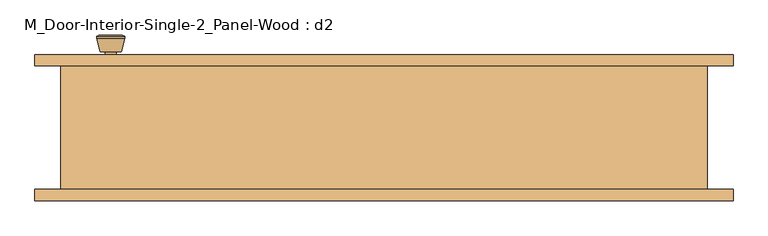
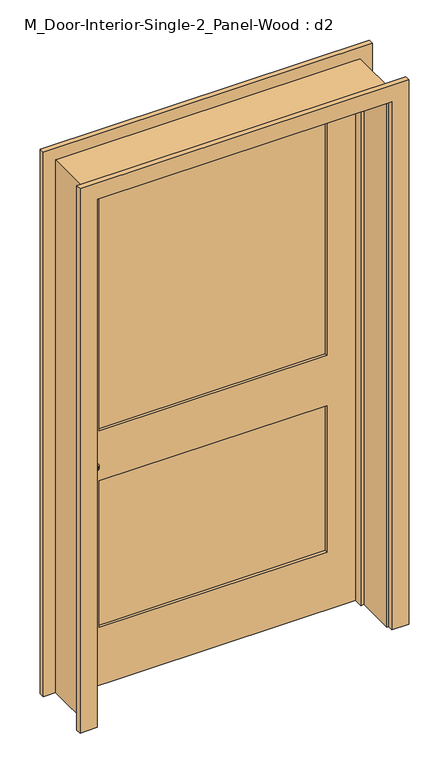
"""IFC4 building model written with IfcOpenShell, lengths in millimetres: door geometry, M_Door-Interior-Single-2_Panel-Wood : d2."""

from ifc_helpers import new_model, si_unit, point, frame, frame_2d, origin, place, context, project, spatial, polyline, circle_curve, trimmed, segment, composite_curve, outline, extrude, faceted_brep, source, transform, mapped, element, save
from ifc_brep_helpers import plane_surface, cylinder_surface, revolved_surface, advanced_brep


def m_door_interior_single_2_panel_wood_d2_7d5fc0ab(model_context):
    return source(origin(), model_context, "Body", "SolidModel", [
        advanced_brep(
        [(-486.5, 65.825, 914.4), (-476.5, 65.825, 914.4), (-496.5, 65.825, 914.4), (-466.0241324, 16.825, 914.4), (-486.5, 16.825, 914.4), (-506.9758676, 16.825, 914.4), (-461.5, 18.6528681, 914.4), (-511.5, 18.6528681, 914.4), (-461.5, 22.1165463, 914.4), (-511.5, 22.1165463, 914.4), (-467.863764, 46.825, 914.4), (-505.136236, 46.825, 914.4), (-476.5, 46.825, 914.4), (-496.5, 46.825, 914.4)],
        [
            (0, 1),
            (1, 2, circle_curve(frame((-486.5, 65.825, 914.4), z_axis=(0.0, 1.0, 0.0), x_axis=(-1.0, 0.0, 0.0)), 10.0)),
            (2, 0),
            (2, 1, circle_curve(frame((-486.5, 65.825, 914.4), z_axis=(0.0, 1.0, 0.0), x_axis=(-1.0, 0.0, 0.0)), 10.0)),
            (3, 4),
            (4, 5),
            (5, 3, circle_curve(frame((-486.5, 16.825, 914.4), z_axis=(0.0, -1.0, 0.0), x_axis=(-1.0, 0.0, 0.0)), 20.4758676)),
            (3, 5, circle_curve(frame((-486.5, 16.825, 914.4), z_axis=(0.0, -1.0, 0.0), x_axis=(-1.0, 0.0, 0.0)), 20.4758676)),
            (6, 3),
            (5, 7),
            (7, 6, circle_curve(frame((-486.5, 18.6528681, 914.4), z_axis=(0.0, -1.0, 0.0), x_axis=(-1.0, 0.0, 0.0)), 25.0)),
            (6, 7, circle_curve(frame((-486.5, 18.6528681, 914.4), z_axis=(0.0, -1.0, 0.0), x_axis=(-1.0, 0.0, 0.0)), 25.0)),
            (8, 6),
            (7, 9),
            (9, 8, circle_curve(frame((-486.5, 22.1165463, 914.4), z_axis=(0.0, -1.0, 0.0), x_axis=(-1.0, 0.0, 0.0)), 25.0)),
            (8, 9, circle_curve(frame((-486.5, 22.1165463, 914.4), z_axis=(0.0, -1.0, 0.0), x_axis=(-1.0, 0.0, 0.0)), 25.0)),
            (10, 8),
            (9, 11),
            (11, 10, circle_curve(frame((-486.5, 46.825, 914.4), z_axis=(0.0, -1.0, 0.0), x_axis=(-1.0, 0.0, 0.0)), 18.636236)),
            (10, 11, circle_curve(frame((-486.5, 46.825, 914.4), z_axis=(0.0, -1.0, 0.0), x_axis=(-1.0, 0.0, 0.0)), 18.636236)),
            (12, 10),
            (11, 13),
            (13, 12, circle_curve(frame((-486.5, 46.825, 914.4), z_axis=(0.0, -1.0, 0.0), x_axis=(-1.0, 0.0, 0.0)), 10.0)),
            (12, 13, circle_curve(frame((-486.5, 46.825, 914.4), z_axis=(0.0, -1.0, 0.0), x_axis=(-1.0, 0.0, 0.0)), 10.0)),
            (1, 12),
            (13, 2),
        ],
        [
            plane_surface(frame((-486.5, 65.825, 914.4), z_axis=(0.0, 1.0, 0.0), x_axis=(-1.0, 0.0, 0.0))),
            plane_surface(frame((-486.5, 16.825, 914.4), z_axis=(0.0, -1.0, 0.0), x_axis=(-1.0, 0.0, 0.0))),
            revolved_surface(polyline([(-506.9758676, 16.825, 914.4), (-511.5, 18.6528681, 914.4)]), (-486.5, 65.825, 914.4), (0.0, 1.0, 0.0)),
            cylinder_surface(frame((-486.5, 65.825, 914.4), z_axis=(0.0, 1.0, 0.0), x_axis=(-1.0, 0.0, 0.0)), 25.0),
            revolved_surface(polyline([(-511.5, 22.1165463, 914.4), (-505.136236, 46.825, 914.4)]), (-486.5, 65.825, 914.4), (0.0, 1.0, 0.0)),
            plane_surface(frame((-486.5, 46.825, 914.4), z_axis=(0.0, 1.0, 0.0), x_axis=(-1.0, 0.0, 0.0))),
            cylinder_surface(frame((-486.5, 65.825, 914.4), z_axis=(0.0, 1.0, 0.0), x_axis=(-1.0, 0.0, 0.0)), 10.0),
        ],
        [
            (0, [[1, 2, 3]]),
            (0, [[-3, 4, -1]]),
            (1, [[5, 6, 7]]),
            (1, [[-6, -5, 8]]),
            (2, [[9, -7, 10, 11]]),
            (2, [[-10, -8, -9, 12]]),
            (3, [[13, -11, 14, 15]]),
            (3, [[-14, -12, -13, 16]]),
            (4, [[17, -15, 18, 19]]),
            (4, [[-18, -16, -17, 20]]),
            (5, [[21, -19, 22, 23]]),
            (5, [[-22, -20, -21, 24]]),
            (6, [[25, -23, 26, -2]]),
            (6, [[-26, -24, -25, -4]]),
        ],
    ),
        extrude(outline(composite_curve([segment(trimmed(circle_curve(frame_2d((914.4, -486.5)), 30.0), [point((914.4, -516.5))], [point((914.4, -456.5))], False, "CARTESIAN"), True, "CONTINUOUS"), segment(trimmed(circle_curve(frame_2d((914.4, -486.5)), 30.0), [point((914.4, -456.5))], [point((914.4, -516.5))], False, "CARTESIAN"), True, "CONTINUOUS")], self_intersect=False)), frame((0.0, 65.825, 0.0), z_axis=(0.0, 1.0, 0.0), x_axis=(0.0, 0.0, 1.0)), (0.0, 0.0, 1.0), 6.0),
        advanced_brep(
        [(-486.5, 112.825, 914.4), (-496.5, 112.825, 914.4), (-476.5, 112.825, 914.4), (-466.0241324, 161.825, 914.4), (-506.9758676, 161.825, 914.4), (-486.5, 161.825, 914.4), (-461.5, 159.9971319, 914.4), (-511.5, 159.9971319, 914.4), (-461.5, 156.5334537, 914.4), (-511.5, 156.5334537, 914.4), (-467.863764, 131.825, 914.4), (-505.136236, 131.825, 914.4), (-476.5, 131.825, 914.4), (-496.5, 131.825, 914.4)],
        [
            (0, 1),
            (1, 2, circle_curve(frame((-486.5, 112.825, 914.4), z_axis=(0.0, -1.0, 0.0), x_axis=(-1.0, 0.0, 0.0)), 10.0)),
            (2, 0),
            (2, 1, circle_curve(frame((-486.5, 112.825, 914.4), z_axis=(0.0, -1.0, 0.0), x_axis=(-1.0, 0.0, 0.0)), 10.0)),
            (3, 4, circle_curve(frame((-486.5, 161.825, 914.4), z_axis=(0.0, 1.0, 0.0), x_axis=(-1.0, 0.0, 0.0)), 20.4758676)),
            (4, 5),
            (5, 3),
            (4, 3, circle_curve(frame((-486.5, 161.825, 914.4), z_axis=(0.0, 1.0, 0.0), x_axis=(-1.0, 0.0, 0.0)), 20.4758676)),
            (6, 7, circle_curve(frame((-486.5, 159.9971319, 914.4), z_axis=(0.0, 1.0, 0.0), x_axis=(-1.0, 0.0, 0.0)), 25.0)),
            (7, 4),
            (3, 6),
            (7, 6, circle_curve(frame((-486.5, 159.9971319, 914.4), z_axis=(0.0, 1.0, 0.0), x_axis=(-1.0, 0.0, 0.0)), 25.0)),
            (8, 9, circle_curve(frame((-486.5, 156.5334537, 914.4), z_axis=(0.0, 1.0, 0.0), x_axis=(-1.0, 0.0, 0.0)), 25.0)),
            (9, 7),
            (6, 8),
            (9, 8, circle_curve(frame((-486.5, 156.5334537, 914.4), z_axis=(0.0, 1.0, 0.0), x_axis=(-1.0, 0.0, 0.0)), 25.0)),
            (10, 11, circle_curve(frame((-486.5, 131.825, 914.4), z_axis=(0.0, 1.0, 0.0), x_axis=(-1.0, 0.0, 0.0)), 18.636236)),
            (11, 9),
            (8, 10),
            (11, 10, circle_curve(frame((-486.5, 131.825, 914.4), z_axis=(0.0, 1.0, 0.0), x_axis=(-1.0, 0.0, 0.0)), 18.636236)),
            (12, 13, circle_curve(frame((-486.5, 131.825, 914.4), z_axis=(0.0, 1.0, 0.0), x_axis=(-1.0, 0.0, 0.0)), 10.0)),
            (13, 11),
            (10, 12),
            (13, 12, circle_curve(frame((-486.5, 131.825, 914.4), z_axis=(0.0, 1.0, 0.0), x_axis=(-1.0, 0.0, 0.0)), 10.0)),
            (1, 13),
            (12, 2),
        ],
        [
            plane_surface(frame((-486.5, 112.825, 914.4), z_axis=(0.0, -1.0, 0.0), x_axis=(-1.0, 0.0, 0.0))),
            plane_surface(frame((-486.5, 161.825, 914.4), z_axis=(0.0, 1.0, 0.0), x_axis=(-1.0, 0.0, 0.0))),
            revolved_surface(polyline([(-506.9758676, 161.825, 914.4), (-511.5, 159.9971319, 914.4)]), (-486.5, 112.825, 914.4), (0.0, -1.0, 0.0)),
            cylinder_surface(frame((-486.5, 112.825, 914.4), z_axis=(0.0, -1.0, 0.0), x_axis=(-1.0, 0.0, 0.0)), 25.0),
            revolved_surface(polyline([(-511.5, 156.5334537, 914.4), (-505.136236, 131.825, 914.4)]), (-486.5, 112.825, 914.4), (0.0, -1.0, 0.0)),
            plane_surface(frame((-486.5, 131.825, 914.4), z_axis=(0.0, -1.0, 0.0), x_axis=(-1.0, 0.0, 0.0))),
            cylinder_surface(frame((-486.5, 112.825, 914.4), z_axis=(0.0, -1.0, 0.0), x_axis=(-1.0, 0.0, 0.0)), 10.0),
        ],
        [
            (0, [[1, 2, 3]]),
            (0, [[-3, 4, -1]]),
            (1, [[5, 6, 7]]),
            (1, [[8, -7, -6]]),
            (2, [[9, 10, -5, 11]]),
            (2, [[12, -11, -8, -10]]),
            (3, [[13, 14, -9, 15]]),
            (3, [[16, -15, -12, -14]]),
            (4, [[17, 18, -13, 19]]),
            (4, [[20, -19, -16, -18]]),
            (5, [[21, 22, -17, 23]]),
            (5, [[24, -23, -20, -22]]),
            (6, [[-2, 25, -21, 26]]),
            (6, [[-4, -26, -24, -25]]),
        ],
    ),
        extrude(outline(composite_curve([segment(trimmed(circle_curve(frame_2d((914.4, -486.5)), 30.0), [point((914.4, -516.5))], [point((914.4, -456.5))], False, "CARTESIAN"), True, "CONTINUOUS"), segment(trimmed(circle_curve(frame_2d((914.4, -486.5)), 30.0), [point((914.4, -456.5))], [point((914.4, -516.5))], False, "CARTESIAN"), True, "CONTINUOUS")], self_intersect=False)), frame((0.0, 106.825, 0.0), z_axis=(0.0, 1.0, 0.0), x_axis=(0.0, 0.0, 1.0)), (0.0, 0.0, 1.0), 6.0),
        extrude(outline(polyline([(430.0, 83.4916667), (-430.0, 83.4916667), (-430.0, 95.1583333), (430.0, 95.1583333), (430.0, 83.4916667)])), frame((0.0, 0.0, 1014.4), z_axis=(0.0, 0.0, 1.0), x_axis=(1.0, 0.0, 0.0)), (0.0, 0.0, 1.0), 965.6),
        extrude(outline(polyline([(430.0, 83.4916667), (-430.0, 83.4916667), (-430.0, 95.1583333), (430.0, 95.1583333), (430.0, 83.4916667)])), frame((0.0, 0.0, 230.0), z_axis=(0.0, 0.0, 1.0), x_axis=(1.0, 0.0, 0.0)), (0.0, 0.0, 1.0), 584.4),
        extrude(outline(polyline([(2100.0, -550.0), (0.0, -550.0), (0.0, 550.0), (2100.0, 550.0), (2100.0, -550.0)]), holes=[polyline([(1980.0, -430.0), (1980.0, 430.0), (1014.4, 430.0), (1014.4, -430.0), (1980.0, -430.0)]), polyline([(814.4, -430.0), (814.4, 430.0), (230.0, 430.0), (230.0, -430.0), (814.4, -430.0)])]), frame((0.0, 71.825, 0.0), z_axis=(0.0, 1.0, 0.0), x_axis=(0.0, 0.0, 1.0)), (0.0, 0.0, 1.0), 35.0),
        faceted_brep([(575.0, 106.825, 0.0), (575.0, -113.175, 0.0), (550.0, -113.175, 0.0), (550.0, 36.9, 0.0), (537.3, 36.9, 0.0), (537.3, 71.825, 0.0), (550.0, 71.825, 0.0), (550.0, 106.825, 0.0), (575.0, 106.825, 2125.0), (575.0, -113.175, 2125.0), (-575.0, -113.175, 2125.0), (-575.0, -113.175, 0.0), (-550.0, -113.175, 0.0), (-550.0, -113.175, 2100.0), (550.0, -113.175, 2100.0), (550.0, 36.9, 2100.0), (-550.0, 36.9, 2100.0), (-550.0, 36.9, 0.0), (-537.3, 36.9, 0.0), (-537.3, 36.9, 2087.3), (537.3, 36.9, 2087.3), (537.3, 71.825, 2087.3), (-537.3, 71.825, 2087.3), (-537.3, 71.825, 0.0), (-550.0, 71.825, 0.0), (-550.0, 71.825, 2100.0), (550.0, 71.825, 2100.0), (550.0, 106.825, 2100.0), (-550.0, 106.825, 2100.0), (-550.0, 106.825, 0.0), (-575.0, 106.825, 0.0), (-575.0, 106.825, 2125.0)], [[[0, 1, 2, 3, 4, 5, 6, 7]], [[1, 0, 8, 9]], [[2, 1, 9, 10, 11, 12, 13, 14]], [[3, 2, 14, 15]], [[4, 3, 15, 16, 17, 18, 19, 20]], [[5, 4, 20, 21]], [[6, 5, 21, 22, 23, 24, 25, 26]], [[7, 6, 26, 27]], [[0, 7, 27, 28, 29, 30, 31, 8]], [[9, 8, 31, 10]], [[15, 14, 13, 16]], [[21, 20, 19, 22]], [[27, 26, 25, 28]], [[30, 29, 24, 23, 18, 17, 12, 11]], [[10, 31, 30, 11]], [[16, 13, 12, 17]], [[22, 19, 18, 23]], [[28, 25, 24, 29]]]),
        extrude(outline(polyline([(0.0, 556.35), (0.0, 621.35), (2171.35, 621.35), (2171.35, -621.35), (0.0, -621.35), (0.0, -556.35), (2106.35, -556.35), (2106.35, 556.35), (0.0, 556.35)])), frame((0.0, -133.175, 0.0), z_axis=(0.0, 1.0, 0.0), x_axis=(0.0, 0.0, 1.0)), (0.0, 0.0, 1.0), 20.0),
        extrude(outline(polyline([(0.0, 556.35), (0.0, 621.35), (2171.35, 621.35), (2171.35, -621.35), (0.0, -621.35), (0.0, -556.35), (2106.35, -556.35), (2106.35, 556.35), (0.0, 556.35)])), frame((0.0, 106.825, 0.0), z_axis=(0.0, 1.0, 0.0), x_axis=(0.0, 0.0, 1.0)), (0.0, 0.0, 1.0), 20.0),
    ])


if __name__ == "__main__":
    model = new_model("IFC4")
    model_context = context("Model", 3, world=origin())
    ifc_project = project(units=[si_unit("LENGTHUNIT", "METRE", prefix="MILLI")], contexts=[model_context])
    site = spatial("IfcSite", under=ifc_project)
    building = spatial("IfcBuilding", under=site)
    placement = place(None, origin())
    m_door_interior_single_2_panel_wood_d2_shape = m_door_interior_single_2_panel_wood_d2_7d5fc0ab(model_context)
    element("IfcDoor", 1, ObjectType="M_Door-Interior-Single-2_Panel-Wood : d2", at=placement, inside=building, context=model_context, shape_type="MappedRepresentation", body=[
        mapped(m_door_interior_single_2_panel_wood_d2_shape, transform((0.0, 0.0, 0.0), x_axis=(1.0, 0.0, 0.0), y_axis=(0.0, 1.0, 0.0), z_axis=(0.0, 0.0, 1.0))),
    ])
    save(model, "model.ifc")

# Revit data of these elements
# Type "M_Door-Interior-Single-2_Panel-Wood : d2"
#   Type Mark = "53"
#   Assembly Code = "C1020300"
#   Analytic Construction = "Wooden"
#   Top Rail = 12 cm
#   Thickness = 3.5 cm
#   Thermal Resistance (R) = 0.455703 (m²·K)/W
#   Swing Angle [instance default] = 90.00°
#   Stiles = 12 cm
#   Rough Width = 115 cm
#   Rough Height = 212.5 cm
#   Lock Rail = 20 cm
#   Height = 210 cm
#   Width = 110 cm
#   Heat Transfer Coefficient (U) = 2.19465 W/(m²·K)
#   Bottom Rail = 23 cm
#   Trim Material = Cherry
#   Panel Material = Cherry
#   Frame Material = Cherry
#   Door Handle Material = Aluminum
#   Visual Light Transmittance = 0
#   Solar Heat Gain Coefficient = 0
#   Wall Closure = (empty or 0)
#   Function = (empty or 0)
# Element 1 (IfcDoor, "M_Door-Interior-Single-2_Panel-Wood : d2")
#   Materials on its faces: "Cherry", "Aluminum"
# Materials
#   "Cherry": class "Wood", colour RGB 226 177 128, transparency 0, Description = "Prunus Serotina", Cost = 0
#   "Aluminum": class "Metal", colour RGB 247 247 247, transparency 0, Description = "Aluminum 6061", Cost = 0
